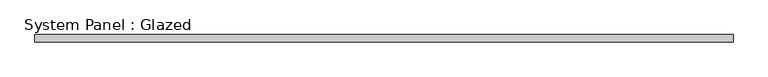
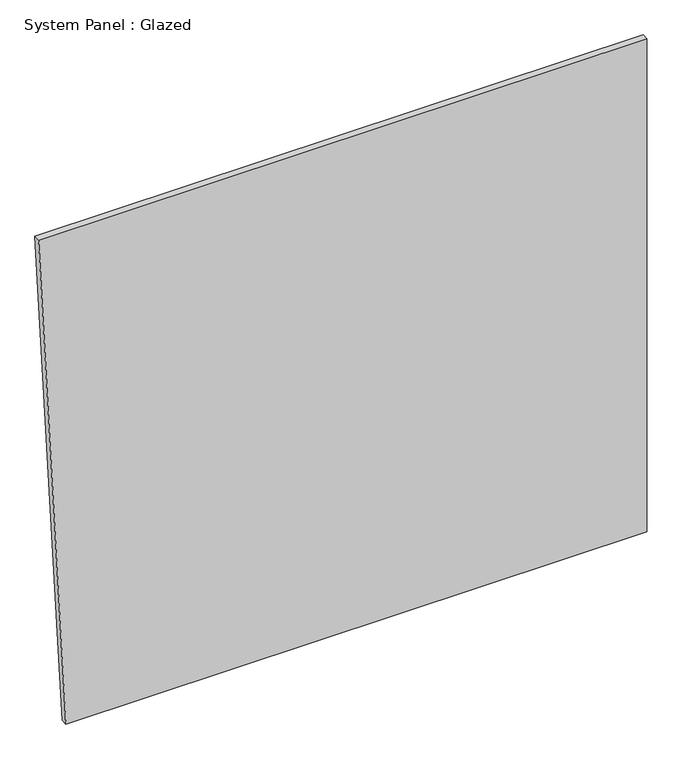
"""IFC4 building model written with IfcOpenShell, lengths in millimetres: plate geometry, System Panel : Glazed."""

import ifcopenshell
import ifcopenshell.guid

model = None  # the IFC model being written
_history = None  # IfcOwnerHistory: only IFC2X3 demands one
_inside = {}  # id of a spatial element -> (the spatial element, [elements in it])
_under = {}  # id of a project, library or spatial element -> (it, [spatial elements below it])
_declared = {}  # id of a project -> (the project, [libraries it declares])
_typed = {}  # id of a type object -> (the type object, [elements of that type])
_made_of = {}  # id of a material, layer set ... -> (it, [elements and type objects made of it])


def new_model(schema):
    """Start an empty IFC model of exactly this schema.

    Asked for "IFC4X3", IfcOpenShell would pick the latest addendum, in which some entities
    have other attributes; the version numbers below select the first issue.
    IFC2X3 requires an IfcOwnerHistory on every rooted entity: one is made here for all.
    """
    global model, _history
    if schema == "IFC4X3":
        model = ifcopenshell.file(schema_version=(4, 3, 0, 0))
    else:
        model = ifcopenshell.file(schema=schema)
    _inside.clear()
    _under.clear()
    _declared.clear()
    _typed.clear()
    _made_of.clear()
    _history = None
    if model.schema == "IFC2X3":
        org = make("IfcOrganization", Name="unknown")
        user = make(
            "IfcPersonAndOrganization",
            ThePerson=make("IfcPerson", FamilyName="unknown"),
            TheOrganization=org,
        )
        app = make(
            "IfcApplication",
            ApplicationDeveloper=org,
            Version="unknown",
            ApplicationFullName="unknown",
            ApplicationIdentifier="unknown",
        )
        _history = make(
            "IfcOwnerHistory",
            OwningUser=user,
            OwningApplication=app,
            ChangeAction="ADDED",
            CreationDate=0,
        )
    return model


def make(cls, **values):
    """One entity of the class cls with the attributes given. An attribute that is None is left unset."""
    return model.create_entity(
        cls, **{name: value for name, value in values.items() if value is not None}
    )


def rooted(cls, **values):
    """An entity with a GlobalId (a new one), such as an element, a storey or a relation."""
    return make(cls, GlobalId=ifcopenshell.guid.new(), OwnerHistory=_history, **values)


def si_unit(unit_type, name, prefix=None):
    """IfcSIUnit, for example si_unit("LENGTHUNIT", "METRE", prefix="MILLI")."""
    return make("IfcSIUnit", UnitType=unit_type, Prefix=prefix, Name=name)


def assignment(units):
    """IfcUnitAssignment: the units of a project."""
    return None if units is None else make("IfcUnitAssignment", Units=units)


def point(xyz):
    """IfcCartesianPoint."""
    return None if xyz is None else make("IfcCartesianPoint", Coordinates=xyz)


def direction(xyz):
    """IfcDirection."""
    return None if xyz is None else make("IfcDirection", DirectionRatios=xyz)


def frame(location, z_axis=None, x_axis=None):
    """IfcAxis2Placement3D, a coordinate frame: its origin and axes. An axis left out is left unset."""
    return make(
        "IfcAxis2Placement3D",
        Location=point(location),
        Axis=direction(z_axis),
        RefDirection=direction(x_axis),
    )


def origin():
    """The frame at (0, 0, 0) with its axes left unset."""
    return frame((0.0, 0.0, 0.0))


def place(relative_to, where):
    """IfcLocalPlacement: puts the frame where relative to a parent placement (None: the world)."""
    return make(
        "IfcLocalPlacement", PlacementRelTo=relative_to, RelativePlacement=where
    )


def context(
    kind, dimensions, precision=None, world=None, true_north=None, identifier=None
):
    """IfcGeometricRepresentationContext, for example the 3D "Model" context."""
    return make(
        "IfcGeometricRepresentationContext",
        ContextIdentifier=identifier,
        ContextType=kind,
        CoordinateSpaceDimension=dimensions,
        Precision=precision,
        WorldCoordinateSystem=world,
        TrueNorth=true_north,
    )


def project(units=None, contexts=None):
    """IfcProject with its units and contexts."""
    return rooted(
        "IfcProject",
        Name="project",
        RepresentationContexts=contexts,
        UnitsInContext=assignment(units),
    )


def spatial(cls, under=None, at=None, **own):
    """A site, building, storey or space (cls), placed at a placement, below another one or the project."""
    s = rooted(cls, ObjectPlacement=at, **own)
    if under is not None:
        _under.setdefault(under.id(), (under, []))[1].append(s)
    return s


def polyline(points):
    """IfcPolyline through the points."""
    return make("IfcPolyline", Points=[point(p) for p in points])


def outline(outer, holes=None, kind="AREA"):
    """IfcArbitraryClosedProfileDef: a profile drawn as a closed curve; with holes, ...WithVoids."""
    if holes is None:
        return make("IfcArbitraryClosedProfileDef", ProfileType=kind, OuterCurve=outer)
    return make(
        "IfcArbitraryProfileDefWithVoids",
        ProfileType=kind,
        OuterCurve=outer,
        InnerCurves=holes,
    )


def extrude(swept, where, along, depth):
    """IfcExtrudedAreaSolid: the profile swept, set in the frame where, extruded along a direction by depth."""
    return make(
        "IfcExtrudedAreaSolid",
        SweptArea=swept,
        Position=where,
        ExtrudedDirection=direction(along),
        Depth=depth,
    )


def shape(context_of_items, identifier, shape_type, items):
    """IfcShapeRepresentation: the items that make up one representation, for example the "Body"."""
    return make(
        "IfcShapeRepresentation",
        ContextOfItems=context_of_items,
        RepresentationIdentifier=identifier,
        RepresentationType=shape_type,
        Items=items,
    )


def source(mapping_origin, context_of_items, identifier, shape_type, items):
    """IfcRepresentationMap: a shape defined once, which mapped items show again and again."""
    return make(
        "IfcRepresentationMap",
        MappingOrigin=mapping_origin,
        MappedRepresentation=shape(context_of_items, identifier, shape_type, items),
    )


def transform(
    local_origin,
    x_axis=None,
    y_axis=None,
    z_axis=None,
    scale=None,
    scale2=None,
    scale3=None,
    uniform=True,
):
    """IfcCartesianTransformationOperator3D, or its non-uniform kind. x_axis, y_axis, z_axis: its Axis1, 2, 3."""
    if uniform:
        return make(
            "IfcCartesianTransformationOperator3D",
            Axis1=direction(x_axis),
            Axis2=direction(y_axis),
            LocalOrigin=point(local_origin),
            Scale=scale,
            Axis3=direction(z_axis),
        )
    return make(
        "IfcCartesianTransformationOperator3DnonUniform",
        Axis1=direction(x_axis),
        Axis2=direction(y_axis),
        LocalOrigin=point(local_origin),
        Scale=scale,
        Axis3=direction(z_axis),
        Scale2=scale2,
        Scale3=scale3,
    )


def mapped(mapping_source, mapping_target):
    """IfcMappedItem: shows the shape of a source again, moved by a transform."""
    return make(
        "IfcMappedItem", MappingSource=mapping_source, MappingTarget=mapping_target
    )


def made_of(thing, what):
    """Note that an element or type object is made of a material, layer set ...; save() writes the relation."""
    if what is not None:
        _made_of.setdefault(what.id(), (what, []))[1].append(thing)
    return thing


def element(
    cls,
    number,
    at=None,
    inside=None,
    cuts=None,
    type_object=None,
    material=None,
    context=None,
    identifier="Body",
    shape_type=None,
    held_by="IfcProductDefinitionShape",
    body=None,
    shapes=None,
    **own,
):
    """One element of the class cls, such as IfcWall. Its Tag is "e" and its number.

    at: its placement. inside: the storey or other place that contains it. cuts: it is an
    opening in that element (IfcRelVoidsElement). A single representation is given by context,
    identifier, shape_type and body (its items); several are given by shapes. held_by: the class
    of the entity that holds the representations. save() writes the other relations.
    """
    e = rooted(cls, Tag="e%d" % number, ObjectPlacement=at, **own)
    if body is not None:
        shapes = [shape(context, identifier, shape_type, body)]
    if shapes is not None:
        e.Representation = make(held_by, Representations=shapes)
    if inside is not None:
        _inside.setdefault(inside.id(), (inside, []))[1].append(e)
    if cuts is not None:
        rooted(
            "IfcRelVoidsElement", RelatingBuildingElement=cuts, RelatedOpeningElement=e
        )
    if type_object is not None:
        _typed.setdefault(type_object.id(), (type_object, []))[1].append(e)
    return made_of(e, material)


def aggregate(whole, parts):
    """IfcRelAggregates: a whole, such as a stair, and the parts it consists of."""
    return rooted("IfcRelAggregates", RelatingObject=whole, RelatedObjects=parts)


def save(model, path):
    """Write the relations noted so far, then the file.

    IfcRelAggregates (storeys below a building ...), IfcRelContainedInSpatialStructure (elements
    in a storey), IfcRelDefinesByType, IfcRelAssociatesMaterial and IfcRelDeclares: one each for
    every whole, place, type object, material and project.
    """
    for whole, parts in _under.values():
        aggregate(whole, parts)
    for where, things in _inside.values():
        rooted(
            "IfcRelContainedInSpatialStructure",
            RelatedElements=things,
            RelatingStructure=where,
        )
    for kind, things in _typed.values():
        rooted("IfcRelDefinesByType", RelatedObjects=things, RelatingType=kind)
    for what, things in _made_of.values():
        rooted("IfcRelAssociatesMaterial", RelatedObjects=things, RelatingMaterial=what)
    for by, libraries in _declared.values():
        rooted("IfcRelDeclares", RelatingContext=by, RelatedDefinitions=libraries)
    model.write(path)


def system_panel_glazed_e065ae4e(model_context):
    return source(origin(), model_context, "Body", "SweptSolid", [
        extrude(outline(polyline([(0.0, -1108.2089886), (0.0, 1217.3908418), (2086.1728929, 1217.3908418), (2086.1728929, -1217.3908418), (0.0, -1108.2089886)])), frame((0.0, -44.45, 0.0), z_axis=(0.0, 1.0, 0.0), x_axis=(0.0, 0.0, 1.0)), (0.0, 0.0, 1.0), 25.4),
    ])


if __name__ == "__main__":
    model = new_model("IFC4")
    model_context = context("Model", 3, world=origin())
    ifc_project = project(units=[si_unit("LENGTHUNIT", "METRE", prefix="MILLI")], contexts=[model_context])
    site = spatial("IfcSite", under=ifc_project)
    building = spatial("IfcBuilding", under=site)
    placement = place(None, origin())
    system_panel_glazed_shape = system_panel_glazed_e065ae4e(model_context)
    element("IfcPlate", 1, ObjectType="System Panel : Glazed", at=placement, inside=building, context=model_context, shape_type="MappedRepresentation", body=[
        mapped(system_panel_glazed_shape, transform((0.0, 0.0, 0.0), x_axis=(1.0, 0.0, 0.0), y_axis=(0.0, 1.0, 0.0), z_axis=(0.0, 0.0, 1.0))),
    ])
    save(model, "model.ifc")

# Revit data of these elements
# Type "System Panel : Glazed"
#   Construction Type Id = "GSP4R"
#   Analytic Construction = "1/8 in Pilkington single glazing"
#   Visual Light Transmittance = 0.9
#   Solar Heat Gain Coefficient = 0.86
#   Heat Transfer Coefficient (U) = 1.18115 BTU/(h·ft²·°F)
#   Define Thermal Properties by = 1
# Element 1 (IfcPlate, "System Panel : Glazed")
#   Materials on its faces: "Glass"
# Materials
#   "Glass": class "Glass", colour RGB 0 128 192, transparency 0.75, Description = "Soda Lime Glass", Cost = 0
